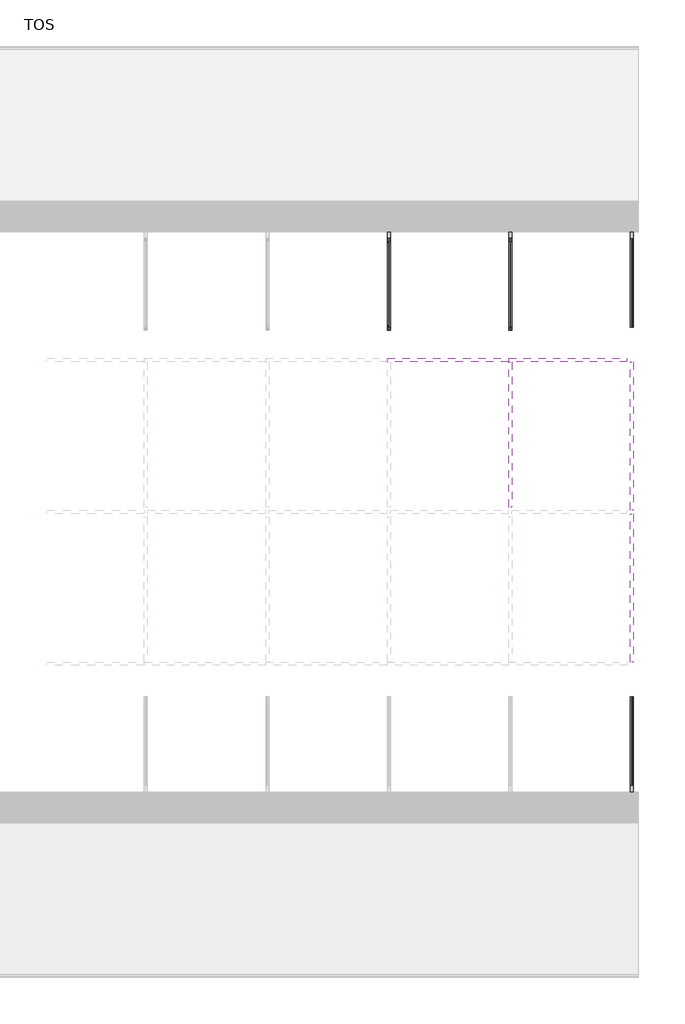
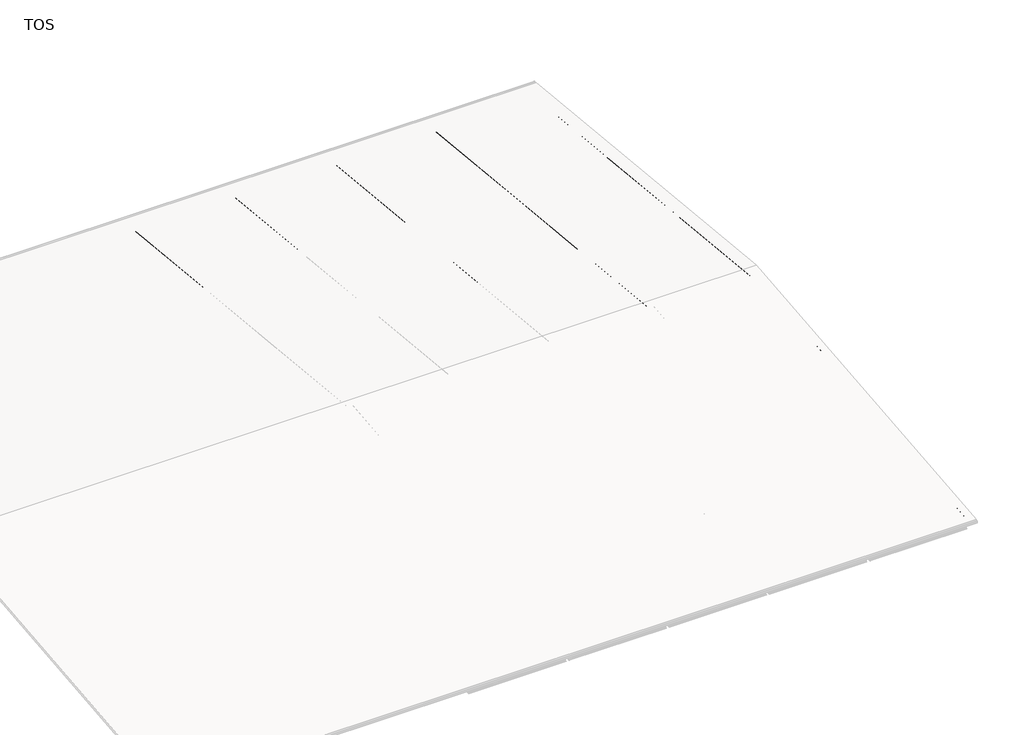
# One storey, part 5 of 5: 23 beams.
"""IFC4 building model written with IfcOpenShell, lengths in millimetres."""

from ifc_helpers import new_model, si_unit, point, frame, frame_2d, origin, place, context, project, spatial, polyline, circle_curve, trimmed, segment, composite_curve, outline, extrude, element, save

model = new_model("IFC4")

# Units and contexts
model_context = context("Model", 3, world=origin())
ifc_project = project(units=[si_unit("LENGTHUNIT", "METRE", prefix="MILLI")], contexts=[model_context])

# Site, building, storey
site = spatial("IfcSite", under=ifc_project)
building = spatial("IfcBuilding", under=site)
storey = spatial("IfcBuildingStorey", under=building, Name="TOS", Elevation=9299.9618634)

# Beams
placement = place(None, origin())
element("IfcBeam", 1, ObjectType="0912_Steel Framing_H-KSD3502 : H_SB_ASB_H-600x200x11x17", at=placement, inside=storey, context=model_context, shape_type="SweptSolid", body=[
    extrude(outline(composite_curve([segment(polyline([(40599.5208589, 10716.9618634), (40599.5208589, 10699.9618634), (40399.5208589, 10699.9618634), (40399.5208589, 10716.9618634), (40472.0208589, 10716.9618634)]), True, "CONTINUOUS"), segment(trimmed(circle_curve(frame_2d((40472.0208589, 10738.9618634)), 22.0), [point((40472.0208589, 10716.9618634))], [point((40494.0208589, 10738.9618634))], True, "CARTESIAN"), True, "CONTINUOUS"), segment(polyline([(40494.0208589, 10738.9618634), (40494.0208589, 11260.9618634)]), True, "CONTINUOUS"), segment(trimmed(circle_curve(frame_2d((40472.0208589, 11260.9618634)), 22.0), [point((40494.0208589, 11260.9618634))], [point((40472.0208589, 11282.9618634))], True, "CARTESIAN"), True, "CONTINUOUS"), segment(polyline([(40472.0208589, 11282.9618634), (40399.5208589, 11282.9618634), (40399.5208589, 11299.9618634), (40599.5208589, 11299.9618634), (40599.5208589, 11282.9618634), (40527.0208589, 11282.9618634)]), True, "CONTINUOUS"), segment(trimmed(circle_curve(frame_2d((40527.0208589, 11260.9618634)), 22.0), [point((40527.0208589, 11282.9618634))], [point((40505.0208589, 11260.9618634))], True, "CARTESIAN"), True, "CONTINUOUS"), segment(polyline([(40505.0208589, 11260.9618634), (40505.0208589, 10738.9618634)]), True, "CONTINUOUS"), segment(trimmed(circle_curve(frame_2d((40527.0208589, 10738.9618634)), 22.0), [point((40505.0208589, 10738.9618634))], [point((40527.0208589, 10716.9618634))], True, "CARTESIAN"), True, "CONTINUOUS"), segment(polyline([(40527.0208589, 10716.9618634), (40599.5208589, 10716.9618634)]), True, "CONTINUOUS")], self_intersect=False)), frame((47900.0, 0.0, 0.0), z_axis=(1.0, 0.0, 0.0), x_axis=(0.0, 1.0, 0.0)), (0.0, 0.0, 1.0), 7987.3),
])
element("IfcBeam", 2, ObjectType="0912_Steel Framing_H-KSD3502 : H_SB_ASB_H-600x200x11x17", at=placement, inside=storey, context=model_context, shape_type="SweptSolid", body=[
    extrude(outline(composite_curve([segment(polyline([(40599.5208589, 10716.9618634), (40599.5208589, 10699.9618634), (40399.5208589, 10699.9618634), (40399.5208589, 10716.9618634), (40472.0208589, 10716.9618634)]), True, "CONTINUOUS"), segment(trimmed(circle_curve(frame_2d((40472.0208589, 10738.9618634)), 22.0), [point((40472.0208589, 10716.9618634))], [point((40494.0208589, 10738.9618634))], True, "CARTESIAN"), True, "CONTINUOUS"), segment(polyline([(40494.0208589, 10738.9618634), (40494.0208589, 11260.9618634)]), True, "CONTINUOUS"), segment(trimmed(circle_curve(frame_2d((40472.0208589, 11260.9618634)), 22.0), [point((40494.0208589, 11260.9618634))], [point((40472.0208589, 11282.9618634))], True, "CARTESIAN"), True, "CONTINUOUS"), segment(polyline([(40472.0208589, 11282.9618634), (40399.5208589, 11282.9618634), (40399.5208589, 11299.9618634), (40599.5208589, 11299.9618634), (40599.5208589, 11282.9618634), (40527.0208589, 11282.9618634)]), True, "CONTINUOUS"), segment(trimmed(circle_curve(frame_2d((40527.0208589, 11260.9618634)), 22.0), [point((40527.0208589, 11282.9618634))], [point((40505.0208589, 11260.9618634))], True, "CARTESIAN"), True, "CONTINUOUS"), segment(polyline([(40505.0208589, 11260.9618634), (40505.0208589, 10738.9618634)]), True, "CONTINUOUS"), segment(trimmed(circle_curve(frame_2d((40527.0208589, 10738.9618634)), 22.0), [point((40505.0208589, 10738.9618634))], [point((40527.0208589, 10716.9618634))], True, "CARTESIAN"), True, "CONTINUOUS"), segment(polyline([(40527.0208589, 10716.9618634), (40599.5208589, 10716.9618634)]), True, "CONTINUOUS")], self_intersect=False)), frame((55900.0, 0.0, 0.0), z_axis=(1.0, 0.0, 0.0), x_axis=(0.0, 1.0, 0.0)), (0.0, 0.0, 1.0), 7781.3),
])
element("IfcBeam", 3, ObjectType="0912_Steel Framing_H-KSD3502 : H_SB_ASB_H-600x200x11x17", at=placement, inside=storey, context=model_context, shape_type="SweptSolid", body=[
    extrude(outline(composite_curve([segment(polyline([(50599.5208589, 9716.9618634), (50599.5208589, 9699.9618634), (50399.5208589, 9699.9618634), (50399.5208589, 9716.9618634), (50472.0208589, 9716.9618634)]), True, "CONTINUOUS"), segment(trimmed(circle_curve(frame_2d((50472.0208589, 9738.9618634)), 22.0), [point((50472.0208589, 9716.9618634))], [point((50494.0208589, 9738.9618634))], True, "CARTESIAN"), True, "CONTINUOUS"), segment(polyline([(50494.0208589, 9738.9618634), (50494.0208589, 10260.9618634)]), True, "CONTINUOUS"), segment(trimmed(circle_curve(frame_2d((50472.0208589, 10260.9618634)), 22.0), [point((50494.0208589, 10260.9618634))], [point((50472.0208589, 10282.9618634))], True, "CARTESIAN"), True, "CONTINUOUS"), segment(polyline([(50472.0208589, 10282.9618634), (50399.5208589, 10282.9618634), (50399.5208589, 10299.9618634), (50599.5208589, 10299.9618634), (50599.5208589, 10282.9618634), (50527.0208589, 10282.9618634)]), True, "CONTINUOUS"), segment(trimmed(circle_curve(frame_2d((50527.0208589, 10260.9618634)), 22.0), [point((50527.0208589, 10282.9618634))], [point((50505.0208589, 10260.9618634))], True, "CARTESIAN"), True, "CONTINUOUS"), segment(polyline([(50505.0208589, 10260.9618634), (50505.0208589, 9738.9618634)]), True, "CONTINUOUS"), segment(trimmed(circle_curve(frame_2d((50527.0208589, 9738.9618634)), 22.0), [point((50505.0208589, 9738.9618634))], [point((50527.0208589, 9716.9618634))], True, "CARTESIAN"), True, "CONTINUOUS"), segment(polyline([(50527.0208589, 9716.9618634), (50599.5208589, 9716.9618634)]), True, "CONTINUOUS")], self_intersect=False)), frame((31900.0, 0.0, 0.0), z_axis=(1.0, 0.0, 0.0), x_axis=(0.0, 1.0, 0.0)), (0.0, 0.0, 1.0), 7987.3),
])
element("IfcBeam", 4, ObjectType="0912_Steel Framing_H-KSD3502 : H_SB_ASB_H-600x200x11x17", at=placement, inside=storey, context=model_context, shape_type="SweptSolid", body=[
    extrude(outline(composite_curve([segment(polyline([(50599.5208589, 9716.9618634), (50599.5208589, 9699.9618634), (50399.5208589, 9699.9618634), (50399.5208589, 9716.9618634), (50472.0208589, 9716.9618634)]), True, "CONTINUOUS"), segment(trimmed(circle_curve(frame_2d((50472.0208589, 9738.9618634)), 22.0), [point((50472.0208589, 9716.9618634))], [point((50494.0208589, 9738.9618634))], True, "CARTESIAN"), True, "CONTINUOUS"), segment(polyline([(50494.0208589, 9738.9618634), (50494.0208589, 10260.9618634)]), True, "CONTINUOUS"), segment(trimmed(circle_curve(frame_2d((50472.0208589, 10260.9618634)), 22.0), [point((50494.0208589, 10260.9618634))], [point((50472.0208589, 10282.9618634))], True, "CARTESIAN"), True, "CONTINUOUS"), segment(polyline([(50472.0208589, 10282.9618634), (50399.5208589, 10282.9618634), (50399.5208589, 10299.9618634), (50599.5208589, 10299.9618634), (50599.5208589, 10282.9618634), (50527.0208589, 10282.9618634)]), True, "CONTINUOUS"), segment(trimmed(circle_curve(frame_2d((50527.0208589, 10260.9618634)), 22.0), [point((50527.0208589, 10282.9618634))], [point((50505.0208589, 10260.9618634))], True, "CARTESIAN"), True, "CONTINUOUS"), segment(polyline([(50505.0208589, 10260.9618634), (50505.0208589, 9738.9618634)]), True, "CONTINUOUS"), segment(trimmed(circle_curve(frame_2d((50527.0208589, 9738.9618634)), 22.0), [point((50505.0208589, 9738.9618634))], [point((50527.0208589, 9716.9618634))], True, "CARTESIAN"), True, "CONTINUOUS"), segment(polyline([(50527.0208589, 9716.9618634), (50599.5208589, 9716.9618634)]), True, "CONTINUOUS")], self_intersect=False)), frame((39900.0, 0.0, 0.0), z_axis=(1.0, 0.0, 0.0), x_axis=(0.0, 1.0, 0.0)), (0.0, 0.0, 1.0), 7987.3),
])
element("IfcBeam", 5, ObjectType="0912_Steel Framing_H-KSD3502 : H_SB_ASB_H-600x200x11x17", at=placement, inside=storey, context=model_context, shape_type="SweptSolid", body=[
    extrude(outline(composite_curve([segment(polyline([(50599.5208589, 9716.9618634), (50599.5208589, 9699.9618634), (50399.5208589, 9699.9618634), (50399.5208589, 9716.9618634), (50472.0208589, 9716.9618634)]), True, "CONTINUOUS"), segment(trimmed(circle_curve(frame_2d((50472.0208589, 9738.9618634)), 22.0), [point((50472.0208589, 9716.9618634))], [point((50494.0208589, 9738.9618634))], True, "CARTESIAN"), True, "CONTINUOUS"), segment(polyline([(50494.0208589, 9738.9618634), (50494.0208589, 10260.9618634)]), True, "CONTINUOUS"), segment(trimmed(circle_curve(frame_2d((50472.0208589, 10260.9618634)), 22.0), [point((50494.0208589, 10260.9618634))], [point((50472.0208589, 10282.9618634))], True, "CARTESIAN"), True, "CONTINUOUS"), segment(polyline([(50472.0208589, 10282.9618634), (50399.5208589, 10282.9618634), (50399.5208589, 10299.9618634), (50599.5208589, 10299.9618634), (50599.5208589, 10282.9618634), (50527.0208589, 10282.9618634)]), True, "CONTINUOUS"), segment(trimmed(circle_curve(frame_2d((50527.0208589, 10260.9618634)), 22.0), [point((50527.0208589, 10282.9618634))], [point((50505.0208589, 10260.9618634))], True, "CARTESIAN"), True, "CONTINUOUS"), segment(polyline([(50505.0208589, 10260.9618634), (50505.0208589, 9738.9618634)]), True, "CONTINUOUS"), segment(trimmed(circle_curve(frame_2d((50527.0208589, 9738.9618634)), 22.0), [point((50505.0208589, 9738.9618634))], [point((50527.0208589, 9716.9618634))], True, "CARTESIAN"), True, "CONTINUOUS"), segment(polyline([(50527.0208589, 9716.9618634), (50599.5208589, 9716.9618634)]), True, "CONTINUOUS")], self_intersect=False)), frame((47900.0, 0.0, 0.0), z_axis=(1.0, 0.0, 0.0), x_axis=(0.0, 1.0, 0.0)), (0.0, 0.0, 1.0), 7987.3),
])
element("IfcBeam", 6, ObjectType="0912_Steel Framing_H-KSD3502 : H_SB_ASB_H-600x200x11x17", at=placement, inside=storey, context=model_context, shape_type="SweptSolid", body=[
    extrude(outline(composite_curve([segment(polyline([(50599.5208589, 9716.9618634), (50599.5208589, 9699.9618634), (50399.5208589, 9699.9618634), (50399.5208589, 9716.9618634), (50472.0208589, 9716.9618634)]), True, "CONTINUOUS"), segment(trimmed(circle_curve(frame_2d((50472.0208589, 9738.9618634)), 22.0), [point((50472.0208589, 9716.9618634))], [point((50494.0208589, 9738.9618634))], True, "CARTESIAN"), True, "CONTINUOUS"), segment(polyline([(50494.0208589, 9738.9618634), (50494.0208589, 10260.9618634)]), True, "CONTINUOUS"), segment(trimmed(circle_curve(frame_2d((50472.0208589, 10260.9618634)), 22.0), [point((50494.0208589, 10260.9618634))], [point((50472.0208589, 10282.9618634))], True, "CARTESIAN"), True, "CONTINUOUS"), segment(polyline([(50472.0208589, 10282.9618634), (50399.5208589, 10282.9618634), (50399.5208589, 10299.9618634), (50599.5208589, 10299.9618634), (50599.5208589, 10282.9618634), (50527.0208589, 10282.9618634)]), True, "CONTINUOUS"), segment(trimmed(circle_curve(frame_2d((50527.0208589, 10260.9618634)), 22.0), [point((50527.0208589, 10282.9618634))], [point((50505.0208589, 10260.9618634))], True, "CARTESIAN"), True, "CONTINUOUS"), segment(polyline([(50505.0208589, 10260.9618634), (50505.0208589, 9738.9618634)]), True, "CONTINUOUS"), segment(trimmed(circle_curve(frame_2d((50527.0208589, 9738.9618634)), 22.0), [point((50505.0208589, 9738.9618634))], [point((50527.0208589, 9716.9618634))], True, "CARTESIAN"), True, "CONTINUOUS"), segment(polyline([(50527.0208589, 9716.9618634), (50599.5208589, 9716.9618634)]), True, "CONTINUOUS")], self_intersect=False)), frame((55900.0, 0.0, 0.0), z_axis=(1.0, 0.0, 0.0), x_axis=(0.0, 1.0, 0.0)), (0.0, 0.0, 1.0), 7781.3),
])
element("IfcBeam", 7, ObjectType="0912_Steel Framing_H-KSD3502 : H_SB_ASB_H-600x200x11x17", at=placement, inside=storey, context=model_context, shape_type="SweptSolid", body=[
    extrude(outline(composite_curve([segment(polyline([(60599.5208589, 8716.9618634), (60599.5208589, 8699.9618634), (60399.5208589, 8699.9618634), (60399.5208589, 8716.9618634), (60472.0208589, 8716.9618634)]), True, "CONTINUOUS"), segment(trimmed(circle_curve(frame_2d((60472.0208589, 8738.9618634)), 22.0), [point((60472.0208589, 8716.9618634))], [point((60494.0208589, 8738.9618634))], True, "CARTESIAN"), True, "CONTINUOUS"), segment(polyline([(60494.0208589, 8738.9618634), (60494.0208589, 9260.9618634)]), True, "CONTINUOUS"), segment(trimmed(circle_curve(frame_2d((60472.0208589, 9260.9618634)), 22.0), [point((60494.0208589, 9260.9618634))], [point((60472.0208589, 9282.9618634))], True, "CARTESIAN"), True, "CONTINUOUS"), segment(polyline([(60472.0208589, 9282.9618634), (60399.5208589, 9282.9618634), (60399.5208589, 9299.9618634), (60599.5208589, 9299.9618634), (60599.5208589, 9282.9618634), (60527.0208589, 9282.9618634)]), True, "CONTINUOUS"), segment(trimmed(circle_curve(frame_2d((60527.0208589, 9260.9618634)), 22.0), [point((60527.0208589, 9282.9618634))], [point((60505.0208589, 9260.9618634))], True, "CARTESIAN"), True, "CONTINUOUS"), segment(polyline([(60505.0208589, 9260.9618634), (60505.0208589, 8738.9618634)]), True, "CONTINUOUS"), segment(trimmed(circle_curve(frame_2d((60527.0208589, 8738.9618634)), 22.0), [point((60505.0208589, 8738.9618634))], [point((60527.0208589, 8716.9618634))], True, "CARTESIAN"), True, "CONTINUOUS"), segment(polyline([(60527.0208589, 8716.9618634), (60599.5208589, 8716.9618634)]), True, "CONTINUOUS")], self_intersect=False)), frame((32113.7, 0.0, 0.0), z_axis=(1.0, 0.0, 0.0), x_axis=(0.0, 1.0, 0.0)), (0.0, 0.0, 1.0), 7772.6),
])
element("IfcBeam", 8, ObjectType="0912_Steel Framing_H-KSD3502 : H_SB_ASB_H-600x200x11x17", at=placement, inside=storey, context=model_context, shape_type="SweptSolid", body=[
    extrude(outline(composite_curve([segment(polyline([(60599.5208589, 8716.9618634), (60599.5208589, 8699.9618634), (60399.5208589, 8699.9618634), (60399.5208589, 8716.9618634), (60472.0208589, 8716.9618634)]), True, "CONTINUOUS"), segment(trimmed(circle_curve(frame_2d((60472.0208589, 8738.9618634)), 22.0), [point((60472.0208589, 8716.9618634))], [point((60494.0208589, 8738.9618634))], True, "CARTESIAN"), True, "CONTINUOUS"), segment(polyline([(60494.0208589, 8738.9618634), (60494.0208589, 9260.9618634)]), True, "CONTINUOUS"), segment(trimmed(circle_curve(frame_2d((60472.0208589, 9260.9618634)), 22.0), [point((60494.0208589, 9260.9618634))], [point((60472.0208589, 9282.9618634))], True, "CARTESIAN"), True, "CONTINUOUS"), segment(polyline([(60472.0208589, 9282.9618634), (60399.5208589, 9282.9618634), (60399.5208589, 9299.9618634), (60599.5208589, 9299.9618634), (60599.5208589, 9282.9618634), (60527.0208589, 9282.9618634)]), True, "CONTINUOUS"), segment(trimmed(circle_curve(frame_2d((60527.0208589, 9260.9618634)), 22.0), [point((60527.0208589, 9282.9618634))], [point((60505.0208589, 9260.9618634))], True, "CARTESIAN"), True, "CONTINUOUS"), segment(polyline([(60505.0208589, 9260.9618634), (60505.0208589, 8738.9618634)]), True, "CONTINUOUS"), segment(trimmed(circle_curve(frame_2d((60527.0208589, 8738.9618634)), 22.0), [point((60505.0208589, 8738.9618634))], [point((60527.0208589, 8716.9618634))], True, "CARTESIAN"), True, "CONTINUOUS"), segment(polyline([(60527.0208589, 8716.9618634), (60599.5208589, 8716.9618634)]), True, "CONTINUOUS")], self_intersect=False)), frame((40113.7, 0.0, 0.0), z_axis=(1.0, 0.0, 0.0), x_axis=(0.0, 1.0, 0.0)), (0.0, 0.0, 1.0), 7772.6),
])
element("IfcBeam", 9, ObjectType="0912_Steel Framing_H-KSD3502 : H_SB_ASB_H-600x200x11x17", at=placement, inside=storey, context=model_context, shape_type="SweptSolid", body=[
    extrude(outline(composite_curve([segment(polyline([(60599.5208589, 8716.9618634), (60599.5208589, 8699.9618634), (60399.5208589, 8699.9618634), (60399.5208589, 8716.9618634), (60472.0208589, 8716.9618634)]), True, "CONTINUOUS"), segment(trimmed(circle_curve(frame_2d((60472.0208589, 8738.9618634)), 22.0), [point((60472.0208589, 8716.9618634))], [point((60494.0208589, 8738.9618634))], True, "CARTESIAN"), True, "CONTINUOUS"), segment(polyline([(60494.0208589, 8738.9618634), (60494.0208589, 9260.9618634)]), True, "CONTINUOUS"), segment(trimmed(circle_curve(frame_2d((60472.0208589, 9260.9618634)), 22.0), [point((60494.0208589, 9260.9618634))], [point((60472.0208589, 9282.9618634))], True, "CARTESIAN"), True, "CONTINUOUS"), segment(polyline([(60472.0208589, 9282.9618634), (60399.5208589, 9282.9618634), (60399.5208589, 9299.9618634), (60599.5208589, 9299.9618634), (60599.5208589, 9282.9618634), (60527.0208589, 9282.9618634)]), True, "CONTINUOUS"), segment(trimmed(circle_curve(frame_2d((60527.0208589, 9260.9618634)), 22.0), [point((60527.0208589, 9282.9618634))], [point((60505.0208589, 9260.9618634))], True, "CARTESIAN"), True, "CONTINUOUS"), segment(polyline([(60505.0208589, 9260.9618634), (60505.0208589, 8738.9618634)]), True, "CONTINUOUS"), segment(trimmed(circle_curve(frame_2d((60527.0208589, 8738.9618634)), 22.0), [point((60505.0208589, 8738.9618634))], [point((60527.0208589, 8716.9618634))], True, "CARTESIAN"), True, "CONTINUOUS"), segment(polyline([(60527.0208589, 8716.9618634), (60599.5208589, 8716.9618634)]), True, "CONTINUOUS")], self_intersect=False)), frame((48113.7, 0.0, 0.0), z_axis=(1.0, 0.0, 0.0), x_axis=(0.0, 1.0, 0.0)), (0.0, 0.0, 1.0), 7772.6),
])
element("IfcBeam", 10, ObjectType="0912_Steel Framing_H-KSD3502 : H_SB_ASB_H-600x200x11x17", at=placement, inside=storey, context=model_context, shape_type="SweptSolid", body=[
    extrude(outline(composite_curve([segment(polyline([(60599.5208589, 8716.9618634), (60599.5208589, 8699.9618634), (60399.5208589, 8699.9618634), (60399.5208589, 8716.9618634), (60472.0208589, 8716.9618634)]), True, "CONTINUOUS"), segment(trimmed(circle_curve(frame_2d((60472.0208589, 8738.9618634)), 22.0), [point((60472.0208589, 8716.9618634))], [point((60494.0208589, 8738.9618634))], True, "CARTESIAN"), True, "CONTINUOUS"), segment(polyline([(60494.0208589, 8738.9618634), (60494.0208589, 9260.9618634)]), True, "CONTINUOUS"), segment(trimmed(circle_curve(frame_2d((60472.0208589, 9260.9618634)), 22.0), [point((60494.0208589, 9260.9618634))], [point((60472.0208589, 9282.9618634))], True, "CARTESIAN"), True, "CONTINUOUS"), segment(polyline([(60472.0208589, 9282.9618634), (60399.5208589, 9282.9618634), (60399.5208589, 9299.9618634), (60599.5208589, 9299.9618634), (60599.5208589, 9282.9618634), (60527.0208589, 9282.9618634)]), True, "CONTINUOUS"), segment(trimmed(circle_curve(frame_2d((60527.0208589, 9260.9618634)), 22.0), [point((60527.0208589, 9282.9618634))], [point((60505.0208589, 9260.9618634))], True, "CARTESIAN"), True, "CONTINUOUS"), segment(polyline([(60505.0208589, 9260.9618634), (60505.0208589, 8738.9618634)]), True, "CONTINUOUS"), segment(trimmed(circle_curve(frame_2d((60527.0208589, 8738.9618634)), 22.0), [point((60505.0208589, 8738.9618634))], [point((60527.0208589, 8716.9618634))], True, "CARTESIAN"), True, "CONTINUOUS"), segment(polyline([(60527.0208589, 8716.9618634), (60599.5208589, 8716.9618634)]), True, "CONTINUOUS")], self_intersect=False)), frame((56113.7, 0.0, 0.0), z_axis=(1.0, 0.0, 0.0), x_axis=(0.0, 1.0, 0.0)), (0.0, 0.0, 1.0), 7772.6),
])
element("IfcBeam", 11, ObjectType="0912_Steel Framing_H-KSD3502 : H_SB_ASB_H-600x200x11x17", at=placement, inside=storey, context=model_context, shape_type="SweptSolid", body=[
    extrude(outline(composite_curve([segment(polyline([(-283.0, 100.0), (-283.0, 27.5)]), True, "CONTINUOUS"), segment(trimmed(circle_curve(frame_2d((-260.9999999, 27.5)), 22.0), [point((-283.0, 27.5))], [point((-260.9999999, 5.5))], True, "CARTESIAN"), True, "CONTINUOUS"), segment(polyline([(-260.9999999, 5.5), (261.0000001, 5.5)]), True, "CONTINUOUS"), segment(trimmed(circle_curve(frame_2d((261.0000001, 27.5)), 22.0), [point((261.0000001, 5.5))], [point((283.0000001, 27.5))], True, "CARTESIAN"), True, "CONTINUOUS"), segment(polyline([(283.0000001, 27.5), (283.0000001, 100.0), (300.0, 100.0), (300.0, -100.0), (283.0000001, -100.0), (283.0000001, -27.5)]), True, "CONTINUOUS"), segment(trimmed(circle_curve(frame_2d((261.0000001, -27.5)), 22.0), [point((283.0000001, -27.5))], [point((261.0000001, -5.5))], True, "CARTESIAN"), True, "CONTINUOUS"), segment(polyline([(261.0000001, -5.5), (-260.9999999, -5.5)]), True, "CONTINUOUS"), segment(trimmed(circle_curve(frame_2d((-260.9999999, -27.5)), 22.0), [point((-260.9999999, -5.5))], [point((-283.0, -27.5))], True, "CARTESIAN"), True, "CONTINUOUS"), segment(polyline([(-283.0, -27.5), (-283.0, -100.0), (-299.9999999, -100.0), (-299.9999999, 100.0), (-283.0, 100.0)]), True, "CONTINUOUS")], self_intersect=False)), frame((32000.0, 60154.0624738, 9033.0114332), z_axis=(0.0, -0.9950371902099892, 0.09950371902099907), x_axis=(0.0, 0.09950371902099907, 0.9950371902099892)), (0.0, 0.0, 1.0), 9560.7882905),
])
element("IfcBeam", 12, ObjectType="0912_Steel Framing_H-KSD3502 : H_SB_ASB_H-600x200x11x17", at=placement, inside=storey, context=model_context, shape_type="SweptSolid", body=[
    extrude(outline(composite_curve([segment(polyline([(-283.0, 100.0), (-283.0, 27.5)]), True, "CONTINUOUS"), segment(trimmed(circle_curve(frame_2d((-260.9999999, 27.5)), 22.0), [point((-283.0, 27.5))], [point((-260.9999999, 5.5))], True, "CARTESIAN"), True, "CONTINUOUS"), segment(polyline([(-260.9999999, 5.5), (261.0000001, 5.5)]), True, "CONTINUOUS"), segment(trimmed(circle_curve(frame_2d((261.0000001, 27.5)), 22.0), [point((261.0000001, 5.5))], [point((283.0000001, 27.5))], True, "CARTESIAN"), True, "CONTINUOUS"), segment(polyline([(283.0000001, 27.5), (283.0000001, 100.0), (300.0, 100.0), (300.0, -100.0), (283.0000001, -100.0), (283.0000001, -27.5)]), True, "CONTINUOUS"), segment(trimmed(circle_curve(frame_2d((261.0000001, -27.5)), 22.0), [point((283.0000001, -27.5))], [point((261.0000001, -5.5))], True, "CARTESIAN"), True, "CONTINUOUS"), segment(polyline([(261.0000001, -5.5), (-260.9999999, -5.5)]), True, "CONTINUOUS"), segment(trimmed(circle_curve(frame_2d((-260.9999999, -27.5)), 22.0), [point((-260.9999999, -5.5))], [point((-283.0, -27.5))], True, "CARTESIAN"), True, "CONTINUOUS"), segment(polyline([(-283.0, -27.5), (-283.0, -100.0), (-299.9999999, -100.0), (-299.9999999, 100.0), (-283.0, 100.0)]), True, "CONTINUOUS")], self_intersect=False)), frame((40000.0, 60154.0624738, 9033.0114332), z_axis=(0.0, -0.9950371902099892, 0.09950371902099907), x_axis=(0.0, 0.09950371902099907, 0.9950371902099892)), (0.0, 0.0, 1.0), 9560.7882905),
])
element("IfcBeam", 13, ObjectType="0912_Steel Framing_H-KSD3502 : H_SB_ASB_H-600x200x11x17", at=placement, inside=storey, context=model_context, shape_type="SweptSolid", body=[
    extrude(outline(composite_curve([segment(polyline([(-283.0, 100.0), (-283.0, 27.5)]), True, "CONTINUOUS"), segment(trimmed(circle_curve(frame_2d((-261.0, 27.5)), 22.0), [point((-283.0, 27.5))], [point((-261.0, 5.5))], True, "CARTESIAN"), True, "CONTINUOUS"), segment(polyline([(-261.0, 5.5), (261.0, 5.5)]), True, "CONTINUOUS"), segment(trimmed(circle_curve(frame_2d((261.0, 27.5)), 22.0), [point((261.0, 5.5))], [point((283.0000001, 27.5))], True, "CARTESIAN"), True, "CONTINUOUS"), segment(polyline([(283.0000001, 27.5), (283.0000001, 100.0), (300.0, 100.0), (300.0, -100.0), (283.0000001, -100.0), (283.0000001, -27.5)]), True, "CONTINUOUS"), segment(trimmed(circle_curve(frame_2d((261.0, -27.5)), 22.0), [point((283.0000001, -27.5))], [point((261.0, -5.5))], True, "CARTESIAN"), True, "CONTINUOUS"), segment(polyline([(261.0, -5.5), (-261.0, -5.5)]), True, "CONTINUOUS"), segment(trimmed(circle_curve(frame_2d((-261.0, -27.5)), 22.0), [point((-261.0, -5.5))], [point((-283.0, -27.5))], True, "CARTESIAN"), True, "CONTINUOUS"), segment(polyline([(-283.0, -27.5), (-283.0, -100.0), (-299.9999999, -100.0), (-299.9999999, 100.0), (-283.0, 100.0)]), True, "CONTINUOUS")], self_intersect=False)), frame((48000.0, 50358.0228699, 10012.6153936), z_axis=(0.0, -0.9950371902099892, 0.09950371902099904), x_axis=(0.0, 0.09950371902099904, 0.9950371902099892)), (0.0, 0.0, 1.0), 9765.7659517),
])
element("IfcBeam", 14, ObjectType="0912_Steel Framing_H-KSD3502 : H_SB_ASB_H-600x200x11x17", at=placement, inside=storey, context=model_context, shape_type="SweptSolid", body=[
    extrude(outline(composite_curve([segment(polyline([(-283.0, 100.0), (-283.0, 27.5)]), True, "CONTINUOUS"), segment(trimmed(circle_curve(frame_2d((-260.9999999, 27.5)), 22.0), [point((-283.0, 27.5))], [point((-260.9999999, 5.5))], True, "CARTESIAN"), True, "CONTINUOUS"), segment(polyline([(-260.9999999, 5.5), (261.0000001, 5.5)]), True, "CONTINUOUS"), segment(trimmed(circle_curve(frame_2d((261.0000001, 27.5)), 22.0), [point((261.0000001, 5.5))], [point((283.0000001, 27.5))], True, "CARTESIAN"), True, "CONTINUOUS"), segment(polyline([(283.0000001, 27.5), (283.0000001, 100.0), (300.0, 100.0), (300.0, -100.0), (283.0000001, -100.0), (283.0000001, -27.5)]), True, "CONTINUOUS"), segment(trimmed(circle_curve(frame_2d((261.0000001, -27.5)), 22.0), [point((283.0000001, -27.5))], [point((261.0000001, -5.5))], True, "CARTESIAN"), True, "CONTINUOUS"), segment(polyline([(261.0000001, -5.5), (-260.9999999, -5.5)]), True, "CONTINUOUS"), segment(trimmed(circle_curve(frame_2d((-260.9999999, -27.5)), 22.0), [point((-260.9999999, -5.5))], [point((-283.0, -27.5))], True, "CARTESIAN"), True, "CONTINUOUS"), segment(polyline([(-283.0, -27.5), (-283.0, -100.0), (-299.9999999, -100.0), (-299.9999999, 100.0), (-283.0, 100.0)]), True, "CONTINUOUS")], self_intersect=False)), frame((48000.0, 60154.0624738, 9033.0114332), z_axis=(0.0, -0.9950371902099892, 0.09950371902099898), x_axis=(0.0, 0.09950371902099898, 0.9950371902099892)), (0.0, 0.0, 1.0), 9560.7882905),
])
element("IfcBeam", 15, ObjectType="0912_Steel Framing_H-KSD3502 : H_SB_ASB_H-600x200x11x17", at=placement, inside=storey, context=model_context, shape_type="SweptSolid", body=[
    extrude(outline(composite_curve([segment(polyline([(-283.0, 100.0), (-283.0, 27.5)]), True, "CONTINUOUS"), segment(trimmed(circle_curve(frame_2d((-261.0, 27.5)), 22.0), [point((-283.0, 27.5))], [point((-261.0, 5.5))], True, "CARTESIAN"), True, "CONTINUOUS"), segment(polyline([(-261.0, 5.5), (261.0, 5.5)]), True, "CONTINUOUS"), segment(trimmed(circle_curve(frame_2d((261.0, 27.5)), 22.0), [point((261.0, 5.5))], [point((283.0000001, 27.5))], True, "CARTESIAN"), True, "CONTINUOUS"), segment(polyline([(283.0000001, 27.5), (283.0000001, 100.0), (300.0, 100.0), (300.0, -100.0), (283.0000001, -100.0), (283.0000001, -27.5)]), True, "CONTINUOUS"), segment(trimmed(circle_curve(frame_2d((261.0, -27.5)), 22.0), [point((283.0000001, -27.5))], [point((261.0, -5.5))], True, "CARTESIAN"), True, "CONTINUOUS"), segment(polyline([(261.0, -5.5), (-261.0, -5.5)]), True, "CONTINUOUS"), segment(trimmed(circle_curve(frame_2d((-261.0, -27.5)), 22.0), [point((-261.0, -5.5))], [point((-283.0, -27.5))], True, "CARTESIAN"), True, "CONTINUOUS"), segment(polyline([(-283.0, -27.5), (-283.0, -100.0), (-299.9999999, -100.0), (-299.9999999, 100.0), (-283.0, 100.0)]), True, "CONTINUOUS")], self_intersect=False)), frame((56000.0, 40358.0228699, 11012.6153936), z_axis=(0.0, -0.9950371902099892, 0.09950371902099896), x_axis=(0.0, 0.09950371902099896, 0.9950371902099892)), (0.0, 0.0, 1.0), 9557.4457081),
])
element("IfcBeam", 16, ObjectType="0912_Steel Framing_H-KSD3502 : H_SB_ASB_H-600x200x11x17", at=placement, inside=storey, context=model_context, shape_type="SweptSolid", body=[
    extrude(outline(composite_curve([segment(polyline([(-283.0, 100.0), (-283.0, 27.5)]), True, "CONTINUOUS"), segment(trimmed(circle_curve(frame_2d((-261.0, 27.5)), 22.0), [point((-283.0, 27.5))], [point((-261.0, 5.5))], True, "CARTESIAN"), True, "CONTINUOUS"), segment(polyline([(-261.0, 5.5), (261.0, 5.5)]), True, "CONTINUOUS"), segment(trimmed(circle_curve(frame_2d((261.0, 27.5)), 22.0), [point((261.0, 5.5))], [point((283.0000001, 27.5))], True, "CARTESIAN"), True, "CONTINUOUS"), segment(polyline([(283.0000001, 27.5), (283.0000001, 100.0), (300.0, 100.0), (300.0, -100.0), (283.0000001, -100.0), (283.0000001, -27.5)]), True, "CONTINUOUS"), segment(trimmed(circle_curve(frame_2d((261.0, -27.5)), 22.0), [point((283.0000001, -27.5))], [point((261.0, -5.5))], True, "CARTESIAN"), True, "CONTINUOUS"), segment(polyline([(261.0, -5.5), (-261.0, -5.5)]), True, "CONTINUOUS"), segment(trimmed(circle_curve(frame_2d((-261.0, -27.5)), 22.0), [point((-261.0, -5.5))], [point((-283.0, -27.5))], True, "CARTESIAN"), True, "CONTINUOUS"), segment(polyline([(-283.0, -27.5), (-283.0, -100.0), (-299.9999999, -100.0), (-299.9999999, 100.0), (-283.0, 100.0)]), True, "CONTINUOUS")], self_intersect=False)), frame((56000.0, 50358.0228699, 10012.6153936), z_axis=(0.0, -0.9950371902099892, 0.09950371902099896), x_axis=(0.0, 0.09950371902099896, 0.9950371902099892)), (0.0, 0.0, 1.0), 9765.7659517),
])
element("IfcBeam", 17, ObjectType="0912_Steel Framing_H-KSD3502 : H_SB_ASB_H-600x200x11x17", at=placement, inside=storey, context=model_context, shape_type="SweptSolid", body=[
    extrude(outline(composite_curve([segment(polyline([(-283.0, 100.0), (-283.0, 27.5)]), True, "CONTINUOUS"), segment(trimmed(circle_curve(frame_2d((-260.9999999, 27.5)), 22.0), [point((-283.0, 27.5))], [point((-260.9999999, 5.5))], True, "CARTESIAN"), True, "CONTINUOUS"), segment(polyline([(-260.9999999, 5.5), (261.0000001, 5.5)]), True, "CONTINUOUS"), segment(trimmed(circle_curve(frame_2d((261.0000001, 27.5)), 22.0), [point((261.0000001, 5.5))], [point((283.0000001, 27.5))], True, "CARTESIAN"), True, "CONTINUOUS"), segment(polyline([(283.0000001, 27.5), (283.0000001, 100.0), (300.0, 100.0), (300.0, -100.0), (283.0000001, -100.0), (283.0000001, -27.5)]), True, "CONTINUOUS"), segment(trimmed(circle_curve(frame_2d((261.0000001, -27.5)), 22.0), [point((283.0000001, -27.5))], [point((261.0000001, -5.5))], True, "CARTESIAN"), True, "CONTINUOUS"), segment(polyline([(261.0000001, -5.5), (-260.9999999, -5.5)]), True, "CONTINUOUS"), segment(trimmed(circle_curve(frame_2d((-260.9999999, -27.5)), 22.0), [point((-260.9999999, -5.5))], [point((-283.0, -27.5))], True, "CARTESIAN"), True, "CONTINUOUS"), segment(polyline([(-283.0, -27.5), (-283.0, -100.0), (-299.9999999, -100.0), (-299.9999999, 100.0), (-283.0, 100.0)]), True, "CONTINUOUS")], self_intersect=False)), frame((56000.0, 60154.0624738, 9033.0114332), z_axis=(0.0, -0.9950371902099892, 0.09950371902099907), x_axis=(0.0, 0.09950371902099907, 0.9950371902099892)), (0.0, 0.0, 1.0), 9560.7882905),
])
element("IfcBeam", 18, ObjectType="0912_Steel Framing_H-KSD3502 : H_SB_ASB_H-600x200x11x17", at=placement, inside=storey, context=model_context, shape_type="SweptSolid", body=[
    extrude(outline(composite_curve([segment(polyline([(-283.0, -100.0), (-299.9999999, -100.0), (-299.9999999, 100.0), (-283.0, 100.0), (-283.0, 27.5)]), True, "CONTINUOUS"), segment(trimmed(circle_curve(frame_2d((-261.0, 27.5)), 22.0), [point((-283.0, 27.5))], [point((-261.0, 5.5))], True, "CARTESIAN"), True, "CONTINUOUS"), segment(polyline([(-261.0, 5.5), (261.0, 5.5)]), True, "CONTINUOUS"), segment(trimmed(circle_curve(frame_2d((261.0, 27.5)), 22.0), [point((261.0, 5.5))], [point((283.0000001, 27.5))], True, "CARTESIAN"), True, "CONTINUOUS"), segment(polyline([(283.0000001, 27.5), (283.0000001, 100.0), (300.0, 100.0), (300.0, -100.0), (283.0000001, -100.0), (283.0000001, -27.5)]), True, "CONTINUOUS"), segment(trimmed(circle_curve(frame_2d((261.0, -27.5)), 22.0), [point((283.0000001, -27.5))], [point((261.0, -5.5))], True, "CARTESIAN"), True, "CONTINUOUS"), segment(polyline([(261.0, -5.5), (-261.0, -5.5)]), True, "CONTINUOUS"), segment(trimmed(circle_curve(frame_2d((-261.0, -27.5)), 22.0), [point((-261.0, -5.5))], [point((-283.0, -27.5))], True, "CARTESIAN"), True, "CONTINUOUS"), segment(polyline([(-283.0, -27.5), (-283.0, -100.0)]), True, "CONTINUOUS")], self_intersect=False)), frame((64000.0, 844.9792439, 9033.0114332), z_axis=(0.0, 0.9950371902099892, 0.0995037190209989), x_axis=(0.0, -0.0995037190209989, 0.9950371902099892)), (0.0, 0.0, 1.0), 9558.4904971),
])
element("IfcBeam", 19, ObjectType="0912_Steel Framing_H-KSD3502 : H_SB_ASB_H-600x200x11x17", at=placement, inside=storey, context=model_context, shape_type="SweptSolid", body=[
    extrude(outline(composite_curve([segment(polyline([(-283.0, -100.0), (-299.9999999, -100.0), (-299.9999999, 100.0), (-283.0, 100.0), (-283.0, 27.5)]), True, "CONTINUOUS"), segment(trimmed(circle_curve(frame_2d((-261.0, 27.5)), 22.0), [point((-283.0, 27.5))], [point((-261.0, 5.5))], True, "CARTESIAN"), True, "CONTINUOUS"), segment(polyline([(-261.0, 5.5), (261.0000001, 5.5)]), True, "CONTINUOUS"), segment(trimmed(circle_curve(frame_2d((261.0000001, 27.5)), 22.0), [point((261.0000001, 5.5))], [point((283.0000001, 27.5))], True, "CARTESIAN"), True, "CONTINUOUS"), segment(polyline([(283.0000001, 27.5), (283.0000001, 100.0), (300.0, 100.0), (300.0, -100.0), (283.0000001, -100.0), (283.0000001, -27.5)]), True, "CONTINUOUS"), segment(trimmed(circle_curve(frame_2d((261.0000001, -27.5)), 22.0), [point((283.0000001, -27.5))], [point((261.0000001, -5.5))], True, "CARTESIAN"), True, "CONTINUOUS"), segment(polyline([(261.0000001, -5.5), (-261.0, -5.5)]), True, "CONTINUOUS"), segment(trimmed(circle_curve(frame_2d((-261.0, -27.5)), 22.0), [point((-261.0, -5.5))], [point((-283.0, -27.5))], True, "CARTESIAN"), True, "CONTINUOUS"), segment(polyline([(-283.0, -27.5), (-283.0, -100.0)]), True, "CONTINUOUS")], self_intersect=False)), frame((64000.0, 10642.0089469, 10012.7144035), z_axis=(0.0, 0.9950371902099892, 0.09950371902099887), x_axis=(0.0, -0.09950371902099887, 0.9950371902099892)), (0.0, 0.0, 1.0), 9762.4731211),
])
element("IfcBeam", 20, ObjectType="0912_Steel Framing_H-KSD3502 : H_SB_ASB_H-600x200x11x17", at=placement, inside=storey, context=model_context, shape_type="SweptSolid", body=[
    extrude(outline(composite_curve([segment(polyline([(-283.0, -100.0), (-299.9999999, -100.0), (-299.9999999, 100.0), (-283.0, 100.0), (-283.0, 27.5)]), True, "CONTINUOUS"), segment(trimmed(circle_curve(frame_2d((-261.0, 27.5)), 22.0), [point((-283.0, 27.5))], [point((-261.0, 5.5))], True, "CARTESIAN"), True, "CONTINUOUS"), segment(polyline([(-261.0, 5.5), (261.0000001, 5.5)]), True, "CONTINUOUS"), segment(trimmed(circle_curve(frame_2d((261.0000001, 27.5)), 22.0), [point((261.0000001, 5.5))], [point((283.0000001, 27.5))], True, "CARTESIAN"), True, "CONTINUOUS"), segment(polyline([(283.0000001, 27.5), (283.0000001, 100.0), (300.0, 100.0), (300.0, -100.0), (283.0000001, -100.0), (283.0000001, -27.5)]), True, "CONTINUOUS"), segment(trimmed(circle_curve(frame_2d((261.0000001, -27.5)), 22.0), [point((283.0000001, -27.5))], [point((261.0000001, -5.5))], True, "CARTESIAN"), True, "CONTINUOUS"), segment(polyline([(261.0000001, -5.5), (-261.0, -5.5)]), True, "CONTINUOUS"), segment(trimmed(circle_curve(frame_2d((-261.0, -27.5)), 22.0), [point((-261.0, -5.5))], [point((-283.0, -27.5))], True, "CARTESIAN"), True, "CONTINUOUS"), segment(polyline([(-283.0, -27.5), (-283.0, -100.0)]), True, "CONTINUOUS")], self_intersect=False)), frame((64000.0, 20642.0089469, 11012.7144035), z_axis=(0.0, 0.9950371902099892, 0.09950371902099896), x_axis=(0.0, -0.09950371902099896, 0.9950371902099892)), (0.0, 0.0, 1.0), 9762.4731211),
])
element("IfcBeam", 21, ObjectType="0912_Steel Framing_H-KSD3502 : H_SB_ASB_H-600x200x11x17", at=placement, inside=storey, context=model_context, shape_type="SweptSolid", body=[
    extrude(outline(composite_curve([segment(polyline([(-283.0, 100.0), (-283.0, 27.5)]), True, "CONTINUOUS"), segment(trimmed(circle_curve(frame_2d((-261.0, 27.5)), 22.0), [point((-283.0, 27.5))], [point((-261.0, 5.5))], True, "CARTESIAN"), True, "CONTINUOUS"), segment(polyline([(-261.0, 5.5), (261.0, 5.5)]), True, "CONTINUOUS"), segment(trimmed(circle_curve(frame_2d((261.0, 27.5)), 22.0), [point((261.0, 5.5))], [point((283.0000001, 27.5))], True, "CARTESIAN"), True, "CONTINUOUS"), segment(polyline([(283.0000001, 27.5), (283.0000001, 100.0), (300.0, 100.0), (300.0, -100.0), (283.0000001, -100.0), (283.0000001, -27.5)]), True, "CONTINUOUS"), segment(trimmed(circle_curve(frame_2d((261.0, -27.5)), 22.0), [point((283.0000001, -27.5))], [point((261.0, -5.5))], True, "CARTESIAN"), True, "CONTINUOUS"), segment(polyline([(261.0, -5.5), (-261.0, -5.5)]), True, "CONTINUOUS"), segment(trimmed(circle_curve(frame_2d((-261.0, -27.5)), 22.0), [point((-261.0, -5.5))], [point((-283.0, -27.5))], True, "CARTESIAN"), True, "CONTINUOUS"), segment(polyline([(-283.0, -27.5), (-283.0, -100.0), (-299.9999999, -100.0), (-299.9999999, 100.0), (-283.0, 100.0)]), True, "CONTINUOUS")], self_intersect=False)), frame((64000.0, 40357.0327709, 11012.7144035), z_axis=(0.0, -0.9950371902099892, 0.09950371902099896), x_axis=(0.0, 0.09950371902099896, 0.9950371902099892)), (0.0, 0.0, 1.0), 9762.4731211),
])
element("IfcBeam", 22, ObjectType="0912_Steel Framing_H-KSD3502 : H_SB_ASB_H-600x200x11x17", at=placement, inside=storey, context=model_context, shape_type="SweptSolid", body=[
    extrude(outline(composite_curve([segment(polyline([(-283.0, 100.0), (-283.0, 27.5)]), True, "CONTINUOUS"), segment(trimmed(circle_curve(frame_2d((-261.0, 27.5)), 22.0), [point((-283.0, 27.5))], [point((-261.0, 5.5))], True, "CARTESIAN"), True, "CONTINUOUS"), segment(polyline([(-261.0, 5.5), (261.0, 5.5)]), True, "CONTINUOUS"), segment(trimmed(circle_curve(frame_2d((261.0, 27.5)), 22.0), [point((261.0, 5.5))], [point((283.0000001, 27.5))], True, "CARTESIAN"), True, "CONTINUOUS"), segment(polyline([(283.0000001, 27.5), (283.0000001, 100.0), (300.0, 100.0), (300.0, -100.0), (283.0000001, -100.0), (283.0000001, -27.5)]), True, "CONTINUOUS"), segment(trimmed(circle_curve(frame_2d((261.0, -27.5)), 22.0), [point((283.0000001, -27.5))], [point((261.0, -5.5))], True, "CARTESIAN"), True, "CONTINUOUS"), segment(polyline([(261.0, -5.5), (-261.0, -5.5)]), True, "CONTINUOUS"), segment(trimmed(circle_curve(frame_2d((-261.0, -27.5)), 22.0), [point((-261.0, -5.5))], [point((-283.0, -27.5))], True, "CARTESIAN"), True, "CONTINUOUS"), segment(polyline([(-283.0, -27.5), (-283.0, -100.0), (-299.9999999, -100.0), (-299.9999999, 100.0), (-283.0, 100.0)]), True, "CONTINUOUS")], self_intersect=False)), frame((64000.0, 50357.0327709, 10012.7144035), z_axis=(0.0, -0.9950371902099892, 0.09950371902099896), x_axis=(0.0, 0.09950371902099896, 0.9950371902099892)), (0.0, 0.0, 1.0), 9762.4731211),
])
element("IfcBeam", 23, ObjectType="0912_Steel Framing_H-KSD3502 : H_SB_ASB_H-600x200x11x17", at=placement, inside=storey, context=model_context, shape_type="SweptSolid", body=[
    extrude(outline(composite_curve([segment(polyline([(-283.0, 100.0), (-283.0, 27.5)]), True, "CONTINUOUS"), segment(trimmed(circle_curve(frame_2d((-260.9999999, 27.5)), 22.0), [point((-283.0, 27.5))], [point((-260.9999999, 5.5))], True, "CARTESIAN"), True, "CONTINUOUS"), segment(polyline([(-260.9999999, 5.5), (261.0000001, 5.5)]), True, "CONTINUOUS"), segment(trimmed(circle_curve(frame_2d((261.0000001, 27.5)), 22.0), [point((261.0000001, 5.5))], [point((283.0000001, 27.5))], True, "CARTESIAN"), True, "CONTINUOUS"), segment(polyline([(283.0000001, 27.5), (283.0000001, 100.0), (300.0, 100.0), (300.0, -100.0), (283.0000001, -100.0), (283.0000001, -27.5)]), True, "CONTINUOUS"), segment(trimmed(circle_curve(frame_2d((261.0000001, -27.5)), 22.0), [point((283.0000001, -27.5))], [point((261.0000001, -5.5))], True, "CARTESIAN"), True, "CONTINUOUS"), segment(polyline([(261.0000001, -5.5), (-260.9999999, -5.5)]), True, "CONTINUOUS"), segment(trimmed(circle_curve(frame_2d((-260.9999999, -27.5)), 22.0), [point((-260.9999999, -5.5))], [point((-283.0, -27.5))], True, "CARTESIAN"), True, "CONTINUOUS"), segment(polyline([(-283.0, -27.5), (-283.0, -100.0), (-299.9999999, -100.0), (-299.9999999, 100.0), (-283.0, 100.0)]), True, "CONTINUOUS")], self_intersect=False)), frame((64000.0, 60154.0624738, 9033.0114332), z_axis=(0.0, -0.9950371902099892, 0.09950371902099898), x_axis=(0.0, 0.09950371902099898, 0.9950371902099892)), (0.0, 0.0, 1.0), 9558.4904971),
])

save(model, "model.ifc")

# Revit data of these elements
# Type "0912_Steel Framing_H-KSD3502 : H_SB_ASB_H-600x200x11x17"
#   Width = 20.0 cm
#   Web Thickness = 1.1 cm
#   Web Fillet = 2.2 cm
#   Warping Constant = 1930000.0 cm⁶
#   W = 0
#   Torsional Moment of Inertia = 91.3724 cm⁴
#   Section Area = 134.4 cm²
#   Plastic Modulus weak axis = 361.0 cm³
#   Plastic Modulus strong axis = 2980.0 cm³
#   Perimeter = 1.94 m²/m
#   Nominal Weight = 106.00 kgf/m
#   Moment of Inertia weak axis = 2280.00 cm⁴
#   Moment of Inertia strong axis = 77600.00 cm⁴
#   Height = 60.0 cm
#   Flange Thickness = 1.7 cm
#   Elastic Modulus weak axis = 228.0 cm³
#   Elastic Modulus strong axis = 2590.0 cm³
#   Centroid Vertical = 30.0 cm
#   Centroid Horizontal = 10.0 cm
#   Ix = 776000000
#   Length [instance default] = 1524 mm
#   Zx = 2980000
#   b = 200 mm
#   h = 600 mm
#   r = 22 mm
#   s = 11 mm
#   t = 17 mm
#   A = 0.01344 m²
#   Structural Material [instance default] = Steel, 45-345
#   Assembly Code = ""
# Elements 1, 2, 3, 4, 5, 6, 7, 8, 9, 10, 11, 12, 13, 14, 15, 16, 17, 18, 19, 20, 21, 22, 23 (IfcBeam, "0912_Steel Framing_H-KSD3502 : H_SB_ASB_H-600x200x11x17")
#   Comments = ""
#   Phase Created = New Construction
#   Materials on its faces: "Steel, 45-345"
# Materials
#   "Steel, 45-345": class "Metal", colour RGB 189 187 185, transparency 0, Description = "Steel 345 MPa", Cost = 0
